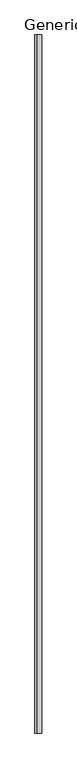
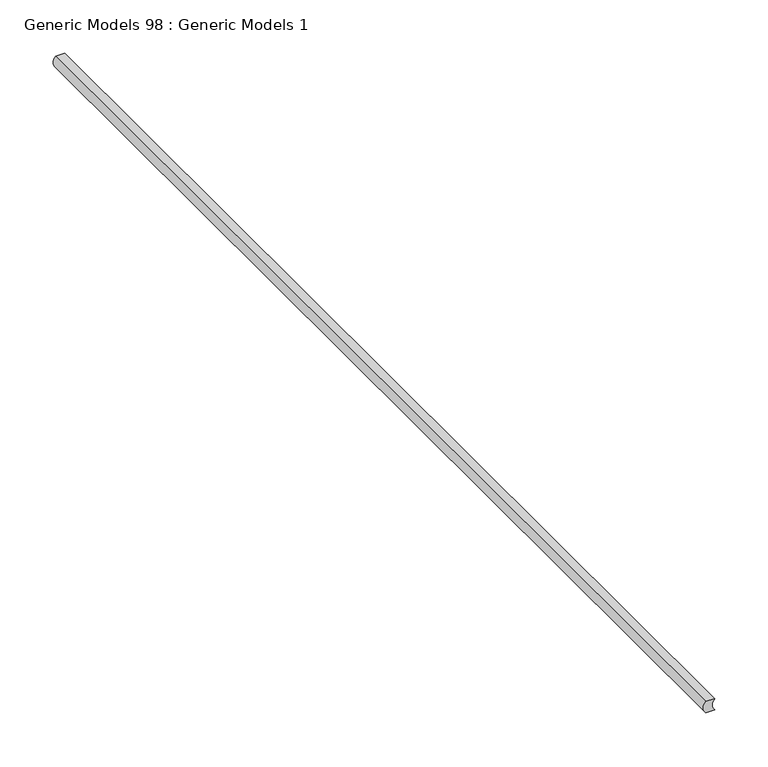
"""IFC4 building model written with IfcOpenShell, lengths in millimetres: proxy geometry, Generic Models 98 : Generic Models 1."""

import ifcopenshell
import ifcopenshell.guid

model = None  # the IFC model being written
_history = None  # IfcOwnerHistory: only IFC2X3 demands one
_inside = {}  # id of a spatial element -> (the spatial element, [elements in it])
_under = {}  # id of a project, library or spatial element -> (it, [spatial elements below it])
_declared = {}  # id of a project -> (the project, [libraries it declares])
_typed = {}  # id of a type object -> (the type object, [elements of that type])
_made_of = {}  # id of a material, layer set ... -> (it, [elements and type objects made of it])


def new_model(schema):
    """Start an empty IFC model of exactly this schema.

    Asked for "IFC4X3", IfcOpenShell would pick the latest addendum, in which some entities
    have other attributes; the version numbers below select the first issue.
    IFC2X3 requires an IfcOwnerHistory on every rooted entity: one is made here for all.
    """
    global model, _history
    if schema == "IFC4X3":
        model = ifcopenshell.file(schema_version=(4, 3, 0, 0))
    else:
        model = ifcopenshell.file(schema=schema)
    _inside.clear()
    _under.clear()
    _declared.clear()
    _typed.clear()
    _made_of.clear()
    _history = None
    if model.schema == "IFC2X3":
        org = make("IfcOrganization", Name="unknown")
        user = make(
            "IfcPersonAndOrganization",
            ThePerson=make("IfcPerson", FamilyName="unknown"),
            TheOrganization=org,
        )
        app = make(
            "IfcApplication",
            ApplicationDeveloper=org,
            Version="unknown",
            ApplicationFullName="unknown",
            ApplicationIdentifier="unknown",
        )
        _history = make(
            "IfcOwnerHistory",
            OwningUser=user,
            OwningApplication=app,
            ChangeAction="ADDED",
            CreationDate=0,
        )
    return model


def make(cls, **values):
    """One entity of the class cls with the attributes given. An attribute that is None is left unset."""
    return model.create_entity(
        cls, **{name: value for name, value in values.items() if value is not None}
    )


def rooted(cls, **values):
    """An entity with a GlobalId (a new one), such as an element, a storey or a relation."""
    return make(cls, GlobalId=ifcopenshell.guid.new(), OwnerHistory=_history, **values)


def si_unit(unit_type, name, prefix=None):
    """IfcSIUnit, for example si_unit("LENGTHUNIT", "METRE", prefix="MILLI")."""
    return make("IfcSIUnit", UnitType=unit_type, Prefix=prefix, Name=name)


def assignment(units):
    """IfcUnitAssignment: the units of a project."""
    return None if units is None else make("IfcUnitAssignment", Units=units)


def point(xyz):
    """IfcCartesianPoint."""
    return None if xyz is None else make("IfcCartesianPoint", Coordinates=xyz)


def direction(xyz):
    """IfcDirection."""
    return None if xyz is None else make("IfcDirection", DirectionRatios=xyz)


def frame(location, z_axis=None, x_axis=None):
    """IfcAxis2Placement3D, a coordinate frame: its origin and axes. An axis left out is left unset."""
    return make(
        "IfcAxis2Placement3D",
        Location=point(location),
        Axis=direction(z_axis),
        RefDirection=direction(x_axis),
    )


def frame_2d(location, x_axis=None):
    """IfcAxis2Placement2D, a coordinate frame in the plane: its origin and x axis."""
    return make(
        "IfcAxis2Placement2D", Location=point(location), RefDirection=direction(x_axis)
    )


def origin():
    """The frame at (0, 0, 0) with its axes left unset."""
    return frame((0.0, 0.0, 0.0))


def place(relative_to, where):
    """IfcLocalPlacement: puts the frame where relative to a parent placement (None: the world)."""
    return make(
        "IfcLocalPlacement", PlacementRelTo=relative_to, RelativePlacement=where
    )


def context(
    kind, dimensions, precision=None, world=None, true_north=None, identifier=None
):
    """IfcGeometricRepresentationContext, for example the 3D "Model" context."""
    return make(
        "IfcGeometricRepresentationContext",
        ContextIdentifier=identifier,
        ContextType=kind,
        CoordinateSpaceDimension=dimensions,
        Precision=precision,
        WorldCoordinateSystem=world,
        TrueNorth=true_north,
    )


def project(units=None, contexts=None):
    """IfcProject with its units and contexts."""
    return rooted(
        "IfcProject",
        Name="project",
        RepresentationContexts=contexts,
        UnitsInContext=assignment(units),
    )


def spatial(cls, under=None, at=None, **own):
    """A site, building, storey or space (cls), placed at a placement, below another one or the project."""
    s = rooted(cls, ObjectPlacement=at, **own)
    if under is not None:
        _under.setdefault(under.id(), (under, []))[1].append(s)
    return s


def polyline(points):
    """IfcPolyline through the points."""
    return make("IfcPolyline", Points=[point(p) for p in points])


def circle_curve(where, radius):
    """IfcCircle in the frame where."""
    return make("IfcCircle", Position=where, Radius=radius)


def trimmed(basis, trim1, trim2, sense, master):
    """IfcTrimmedCurve: the piece of a basis curve between two trims."""
    return make(
        "IfcTrimmedCurve",
        BasisCurve=basis,
        Trim1=trim1,
        Trim2=trim2,
        SenseAgreement=sense,
        MasterRepresentation=master,
    )


def segment(curve, same_sense, transition):
    """IfcCompositeCurveSegment."""
    return make(
        "IfcCompositeCurveSegment",
        Transition=transition,
        SameSense=same_sense,
        ParentCurve=curve,
    )


def composite_curve(segments, self_intersect=None):
    """IfcCompositeCurve: segments joined end to end."""
    return make("IfcCompositeCurve", Segments=segments, SelfIntersect=self_intersect)


def outline(outer, holes=None, kind="AREA"):
    """IfcArbitraryClosedProfileDef: a profile drawn as a closed curve; with holes, ...WithVoids."""
    if holes is None:
        return make("IfcArbitraryClosedProfileDef", ProfileType=kind, OuterCurve=outer)
    return make(
        "IfcArbitraryProfileDefWithVoids",
        ProfileType=kind,
        OuterCurve=outer,
        InnerCurves=holes,
    )


def extrude(swept, where, along, depth):
    """IfcExtrudedAreaSolid: the profile swept, set in the frame where, extruded along a direction by depth."""
    return make(
        "IfcExtrudedAreaSolid",
        SweptArea=swept,
        Position=where,
        ExtrudedDirection=direction(along),
        Depth=depth,
    )


def shape(context_of_items, identifier, shape_type, items):
    """IfcShapeRepresentation: the items that make up one representation, for example the "Body"."""
    return make(
        "IfcShapeRepresentation",
        ContextOfItems=context_of_items,
        RepresentationIdentifier=identifier,
        RepresentationType=shape_type,
        Items=items,
    )


def source(mapping_origin, context_of_items, identifier, shape_type, items):
    """IfcRepresentationMap: a shape defined once, which mapped items show again and again."""
    return make(
        "IfcRepresentationMap",
        MappingOrigin=mapping_origin,
        MappedRepresentation=shape(context_of_items, identifier, shape_type, items),
    )


def transform(
    local_origin,
    x_axis=None,
    y_axis=None,
    z_axis=None,
    scale=None,
    scale2=None,
    scale3=None,
    uniform=True,
):
    """IfcCartesianTransformationOperator3D, or its non-uniform kind. x_axis, y_axis, z_axis: its Axis1, 2, 3."""
    if uniform:
        return make(
            "IfcCartesianTransformationOperator3D",
            Axis1=direction(x_axis),
            Axis2=direction(y_axis),
            LocalOrigin=point(local_origin),
            Scale=scale,
            Axis3=direction(z_axis),
        )
    return make(
        "IfcCartesianTransformationOperator3DnonUniform",
        Axis1=direction(x_axis),
        Axis2=direction(y_axis),
        LocalOrigin=point(local_origin),
        Scale=scale,
        Axis3=direction(z_axis),
        Scale2=scale2,
        Scale3=scale3,
    )


def mapped(mapping_source, mapping_target):
    """IfcMappedItem: shows the shape of a source again, moved by a transform."""
    return make(
        "IfcMappedItem", MappingSource=mapping_source, MappingTarget=mapping_target
    )


def made_of(thing, what):
    """Note that an element or type object is made of a material, layer set ...; save() writes the relation."""
    if what is not None:
        _made_of.setdefault(what.id(), (what, []))[1].append(thing)
    return thing


def element(
    cls,
    number,
    at=None,
    inside=None,
    cuts=None,
    type_object=None,
    material=None,
    context=None,
    identifier="Body",
    shape_type=None,
    held_by="IfcProductDefinitionShape",
    body=None,
    shapes=None,
    **own,
):
    """One element of the class cls, such as IfcWall. Its Tag is "e" and its number.

    at: its placement. inside: the storey or other place that contains it. cuts: it is an
    opening in that element (IfcRelVoidsElement). A single representation is given by context,
    identifier, shape_type and body (its items); several are given by shapes. held_by: the class
    of the entity that holds the representations. save() writes the other relations.
    """
    e = rooted(cls, Tag="e%d" % number, ObjectPlacement=at, **own)
    if body is not None:
        shapes = [shape(context, identifier, shape_type, body)]
    if shapes is not None:
        e.Representation = make(held_by, Representations=shapes)
    if inside is not None:
        _inside.setdefault(inside.id(), (inside, []))[1].append(e)
    if cuts is not None:
        rooted(
            "IfcRelVoidsElement", RelatingBuildingElement=cuts, RelatedOpeningElement=e
        )
    if type_object is not None:
        _typed.setdefault(type_object.id(), (type_object, []))[1].append(e)
    return made_of(e, material)


def aggregate(whole, parts):
    """IfcRelAggregates: a whole, such as a stair, and the parts it consists of."""
    return rooted("IfcRelAggregates", RelatingObject=whole, RelatedObjects=parts)


def save(model, path):
    """Write the relations noted so far, then the file.

    IfcRelAggregates (storeys below a building ...), IfcRelContainedInSpatialStructure (elements
    in a storey), IfcRelDefinesByType, IfcRelAssociatesMaterial and IfcRelDeclares: one each for
    every whole, place, type object, material and project.
    """
    for whole, parts in _under.values():
        aggregate(whole, parts)
    for where, things in _inside.values():
        rooted(
            "IfcRelContainedInSpatialStructure",
            RelatedElements=things,
            RelatingStructure=where,
        )
    for kind, things in _typed.values():
        rooted("IfcRelDefinesByType", RelatedObjects=things, RelatingType=kind)
    for what, things in _made_of.values():
        rooted("IfcRelAssociatesMaterial", RelatedObjects=things, RelatingMaterial=what)
    for by, libraries in _declared.values():
        rooted("IfcRelDeclares", RelatingContext=by, RelatedDefinitions=libraries)
    model.write(path)


def generic_models_98_generic_models_1_309ea474(model_context):
    return source(origin(), model_context, "Body", "SweptSolid", [
        extrude(outline(composite_curve([segment(trimmed(circle_curve(frame_2d((2225.123933, 46957.578034)), 8.620055), [point((2218.773933, 46951.7485531))], [point((2231.473933, 46951.7485531))], True, "CARTESIAN"), True, "CONTINUOUS"), segment(polyline([(2231.473933, 46951.7485531), (2231.473933, 46942.2235531)]), True, "CONTINUOUS"), segment(trimmed(circle_curve(frame_2d((2225.123933, 46948.053034)), 8.620055), [point((2231.473933, 46942.2235531))], [point((2218.773933, 46942.2235531))], False, "CARTESIAN"), True, "CONTINUOUS"), segment(polyline([(2218.773933, 46942.2235531), (2218.773933, 46951.7485531)]), True, "CONTINUOUS")], self_intersect=False)), frame((0.0, 0.0, 0.0), z_axis=(0.0, 1.0, 0.0), x_axis=(0.0, 0.0, 1.0)), (0.0, 0.0, 1.0), 1219.2),
    ])


if __name__ == "__main__":
    model = new_model("IFC4")
    model_context = context("Model", 3, world=origin())
    ifc_project = project(units=[si_unit("LENGTHUNIT", "METRE", prefix="MILLI")], contexts=[model_context])
    site = spatial("IfcSite", under=ifc_project)
    building = spatial("IfcBuilding", under=site)
    placement = place(None, origin())
    generic_models_98_generic_models_1_shape = generic_models_98_generic_models_1_309ea474(model_context)
    element("IfcBuildingElementProxy", 1, Name="Generic Models 98 : Generic Models 1", ObjectType="Generic Models 98 : Generic Models 1", at=placement, inside=building, context=model_context, shape_type="MappedRepresentation", body=[
        mapped(generic_models_98_generic_models_1_shape, transform((0.0, 0.0, 0.0), x_axis=(1.0, 0.0, 0.0), y_axis=(0.0, 1.0, 0.0), z_axis=(0.0, 0.0, 1.0))),
    ])
    save(model, "model.ifc")

# Revit data of these elements
# Element 1 (IfcBuildingElementProxy, "Generic Models 98 : Generic Models 1")
#   Materials on its faces: "SEALANT (W/ BACKER ROD IF NECESSARY)"
# Materials
#   "SEALANT (W/ BACKER ROD IF NECESSARY)": class "Unassigned", colour RGB 120 120 120, transparency 0, Cost = 0
